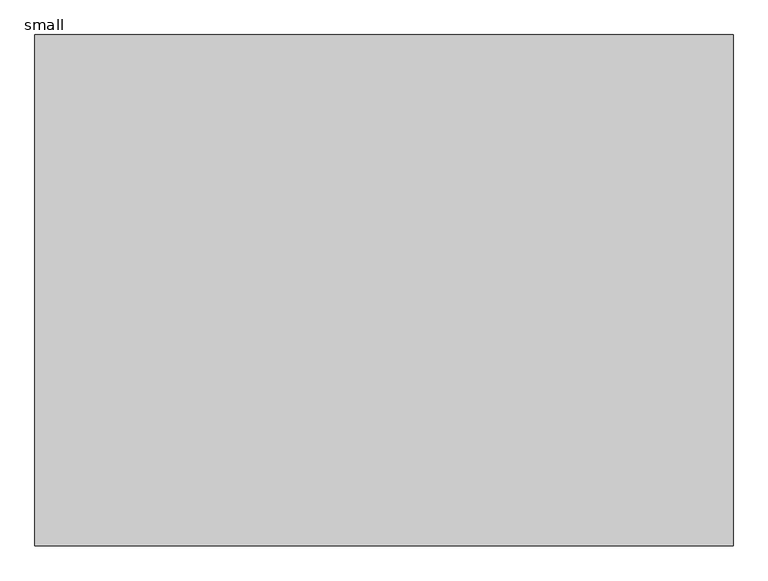
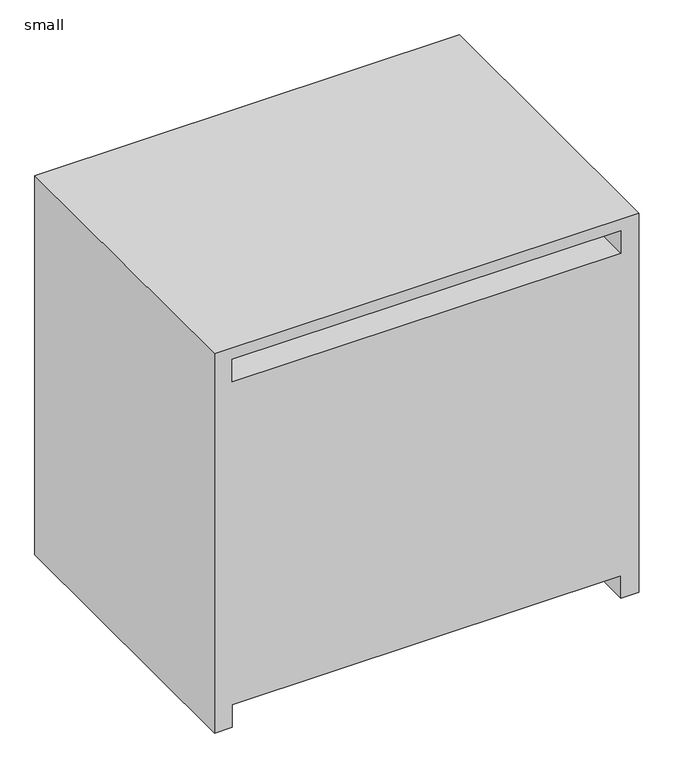
"""IFC4 building model written with IfcOpenShell, lengths in millimetres: proxy geometry, Transformer-Dry-Type-Siemens : small."""

import ifcopenshell
import ifcopenshell.guid

model = None  # the IFC model being written
_history = None  # IfcOwnerHistory: only IFC2X3 demands one
_inside = {}  # id of a spatial element -> (the spatial element, [elements in it])
_under = {}  # id of a project, library or spatial element -> (it, [spatial elements below it])
_declared = {}  # id of a project -> (the project, [libraries it declares])
_typed = {}  # id of a type object -> (the type object, [elements of that type])
_made_of = {}  # id of a material, layer set ... -> (it, [elements and type objects made of it])


def new_model(schema):
    """Start an empty IFC model of exactly this schema.

    Asked for "IFC4X3", IfcOpenShell would pick the latest addendum, in which some entities
    have other attributes; the version numbers below select the first issue.
    IFC2X3 requires an IfcOwnerHistory on every rooted entity: one is made here for all.
    """
    global model, _history
    if schema == "IFC4X3":
        model = ifcopenshell.file(schema_version=(4, 3, 0, 0))
    else:
        model = ifcopenshell.file(schema=schema)
    _inside.clear()
    _under.clear()
    _declared.clear()
    _typed.clear()
    _made_of.clear()
    _history = None
    if model.schema == "IFC2X3":
        org = make("IfcOrganization", Name="unknown")
        user = make(
            "IfcPersonAndOrganization",
            ThePerson=make("IfcPerson", FamilyName="unknown"),
            TheOrganization=org,
        )
        app = make(
            "IfcApplication",
            ApplicationDeveloper=org,
            Version="unknown",
            ApplicationFullName="unknown",
            ApplicationIdentifier="unknown",
        )
        _history = make(
            "IfcOwnerHistory",
            OwningUser=user,
            OwningApplication=app,
            ChangeAction="ADDED",
            CreationDate=0,
        )
    return model


def make(cls, **values):
    """One entity of the class cls with the attributes given. An attribute that is None is left unset."""
    return model.create_entity(
        cls, **{name: value for name, value in values.items() if value is not None}
    )


def rooted(cls, **values):
    """An entity with a GlobalId (a new one), such as an element, a storey or a relation."""
    return make(cls, GlobalId=ifcopenshell.guid.new(), OwnerHistory=_history, **values)


def si_unit(unit_type, name, prefix=None):
    """IfcSIUnit, for example si_unit("LENGTHUNIT", "METRE", prefix="MILLI")."""
    return make("IfcSIUnit", UnitType=unit_type, Prefix=prefix, Name=name)


def assignment(units):
    """IfcUnitAssignment: the units of a project."""
    return None if units is None else make("IfcUnitAssignment", Units=units)


def point(xyz):
    """IfcCartesianPoint."""
    return None if xyz is None else make("IfcCartesianPoint", Coordinates=xyz)


def direction(xyz):
    """IfcDirection."""
    return None if xyz is None else make("IfcDirection", DirectionRatios=xyz)


def frame(location, z_axis=None, x_axis=None):
    """IfcAxis2Placement3D, a coordinate frame: its origin and axes. An axis left out is left unset."""
    return make(
        "IfcAxis2Placement3D",
        Location=point(location),
        Axis=direction(z_axis),
        RefDirection=direction(x_axis),
    )


def origin():
    """The frame at (0, 0, 0) with its axes left unset."""
    return frame((0.0, 0.0, 0.0))


def place(relative_to, where):
    """IfcLocalPlacement: puts the frame where relative to a parent placement (None: the world)."""
    return make(
        "IfcLocalPlacement", PlacementRelTo=relative_to, RelativePlacement=where
    )


def context(
    kind, dimensions, precision=None, world=None, true_north=None, identifier=None
):
    """IfcGeometricRepresentationContext, for example the 3D "Model" context."""
    return make(
        "IfcGeometricRepresentationContext",
        ContextIdentifier=identifier,
        ContextType=kind,
        CoordinateSpaceDimension=dimensions,
        Precision=precision,
        WorldCoordinateSystem=world,
        TrueNorth=true_north,
    )


def project(units=None, contexts=None):
    """IfcProject with its units and contexts."""
    return rooted(
        "IfcProject",
        Name="project",
        RepresentationContexts=contexts,
        UnitsInContext=assignment(units),
    )


def spatial(cls, under=None, at=None, **own):
    """A site, building, storey or space (cls), placed at a placement, below another one or the project."""
    s = rooted(cls, ObjectPlacement=at, **own)
    if under is not None:
        _under.setdefault(under.id(), (under, []))[1].append(s)
    return s


def polyline(points):
    """IfcPolyline through the points."""
    return make("IfcPolyline", Points=[point(p) for p in points])


def outline(outer, holes=None, kind="AREA"):
    """IfcArbitraryClosedProfileDef: a profile drawn as a closed curve; with holes, ...WithVoids."""
    if holes is None:
        return make("IfcArbitraryClosedProfileDef", ProfileType=kind, OuterCurve=outer)
    return make(
        "IfcArbitraryProfileDefWithVoids",
        ProfileType=kind,
        OuterCurve=outer,
        InnerCurves=holes,
    )


def extrude(swept, where, along, depth):
    """IfcExtrudedAreaSolid: the profile swept, set in the frame where, extruded along a direction by depth."""
    return make(
        "IfcExtrudedAreaSolid",
        SweptArea=swept,
        Position=where,
        ExtrudedDirection=direction(along),
        Depth=depth,
    )


def shape(context_of_items, identifier, shape_type, items):
    """IfcShapeRepresentation: the items that make up one representation, for example the "Body"."""
    return make(
        "IfcShapeRepresentation",
        ContextOfItems=context_of_items,
        RepresentationIdentifier=identifier,
        RepresentationType=shape_type,
        Items=items,
    )


def source(mapping_origin, context_of_items, identifier, shape_type, items):
    """IfcRepresentationMap: a shape defined once, which mapped items show again and again."""
    return make(
        "IfcRepresentationMap",
        MappingOrigin=mapping_origin,
        MappedRepresentation=shape(context_of_items, identifier, shape_type, items),
    )


def transform(
    local_origin,
    x_axis=None,
    y_axis=None,
    z_axis=None,
    scale=None,
    scale2=None,
    scale3=None,
    uniform=True,
):
    """IfcCartesianTransformationOperator3D, or its non-uniform kind. x_axis, y_axis, z_axis: its Axis1, 2, 3."""
    if uniform:
        return make(
            "IfcCartesianTransformationOperator3D",
            Axis1=direction(x_axis),
            Axis2=direction(y_axis),
            LocalOrigin=point(local_origin),
            Scale=scale,
            Axis3=direction(z_axis),
        )
    return make(
        "IfcCartesianTransformationOperator3DnonUniform",
        Axis1=direction(x_axis),
        Axis2=direction(y_axis),
        LocalOrigin=point(local_origin),
        Scale=scale,
        Axis3=direction(z_axis),
        Scale2=scale2,
        Scale3=scale3,
    )


def mapped(mapping_source, mapping_target):
    """IfcMappedItem: shows the shape of a source again, moved by a transform."""
    return make(
        "IfcMappedItem", MappingSource=mapping_source, MappingTarget=mapping_target
    )


def made_of(thing, what):
    """Note that an element or type object is made of a material, layer set ...; save() writes the relation."""
    if what is not None:
        _made_of.setdefault(what.id(), (what, []))[1].append(thing)
    return thing


def element(
    cls,
    number,
    at=None,
    inside=None,
    cuts=None,
    type_object=None,
    material=None,
    context=None,
    identifier="Body",
    shape_type=None,
    held_by="IfcProductDefinitionShape",
    body=None,
    shapes=None,
    **own,
):
    """One element of the class cls, such as IfcWall. Its Tag is "e" and its number.

    at: its placement. inside: the storey or other place that contains it. cuts: it is an
    opening in that element (IfcRelVoidsElement). A single representation is given by context,
    identifier, shape_type and body (its items); several are given by shapes. held_by: the class
    of the entity that holds the representations. save() writes the other relations.
    """
    e = rooted(cls, Tag="e%d" % number, ObjectPlacement=at, **own)
    if body is not None:
        shapes = [shape(context, identifier, shape_type, body)]
    if shapes is not None:
        e.Representation = make(held_by, Representations=shapes)
    if inside is not None:
        _inside.setdefault(inside.id(), (inside, []))[1].append(e)
    if cuts is not None:
        rooted(
            "IfcRelVoidsElement", RelatingBuildingElement=cuts, RelatedOpeningElement=e
        )
    if type_object is not None:
        _typed.setdefault(type_object.id(), (type_object, []))[1].append(e)
    return made_of(e, material)


def aggregate(whole, parts):
    """IfcRelAggregates: a whole, such as a stair, and the parts it consists of."""
    return rooted("IfcRelAggregates", RelatingObject=whole, RelatedObjects=parts)


def save(model, path):
    """Write the relations noted so far, then the file.

    IfcRelAggregates (storeys below a building ...), IfcRelContainedInSpatialStructure (elements
    in a storey), IfcRelDefinesByType, IfcRelAssociatesMaterial and IfcRelDeclares: one each for
    every whole, place, type object, material and project.
    """
    for whole, parts in _under.values():
        aggregate(whole, parts)
    for where, things in _inside.values():
        rooted(
            "IfcRelContainedInSpatialStructure",
            RelatedElements=things,
            RelatingStructure=where,
        )
    for kind, things in _typed.values():
        rooted("IfcRelDefinesByType", RelatedObjects=things, RelatingType=kind)
    for what, things in _made_of.values():
        rooted("IfcRelAssociatesMaterial", RelatedObjects=things, RelatingMaterial=what)
    for by, libraries in _declared.values():
        rooted("IfcRelDeclares", RelatingContext=by, RelatedDefinitions=libraries)
    model.write(path)


def small_32f65543(model_context):
    return source(origin(), model_context, "Body", "SweptSolid", [
        extrude(outline(polyline([(1701.8, 901.7), (1701.8, -901.7), (0.0, -901.7), (0.0, -825.5), (101.6, -825.5), (101.6, 825.5), (0.0, 825.5), (0.0, 901.7), (1701.8, 901.7)]), holes=[polyline([(1651.0, 825.5), (1549.4, 825.5), (1549.4, -825.5), (1651.0, -825.5), (1651.0, 825.5)])]), frame((0.0, -660.4, 0.0), z_axis=(0.0, 1.0, 0.0), x_axis=(0.0, 0.0, 1.0)), (0.0, 0.0, 1.0), 1320.8),
    ])


if __name__ == "__main__":
    model = new_model("IFC4")
    model_context = context("Model", 3, world=origin())
    ifc_project = project(units=[si_unit("LENGTHUNIT", "METRE", prefix="MILLI")], contexts=[model_context])
    site = spatial("IfcSite", under=ifc_project)
    building = spatial("IfcBuilding", under=site)
    placement = place(None, origin())
    small_shape = small_32f65543(model_context)
    element("IfcBuildingElementProxy", 1, Name="Transformer-Dry-Type-Siemens : small", ObjectType="Transformer-Dry-Type-Siemens : small", at=placement, inside=building, context=model_context, shape_type="MappedRepresentation", body=[
        mapped(small_shape, transform((0.0, 0.0, 0.0), x_axis=(1.0, 0.0, 0.0), y_axis=(0.0, 1.0, 0.0), z_axis=(0.0, 0.0, 1.0))),
    ])
    save(model, "model.ifc")

# Revit data of these elements
# Type "Transformer-Dry-Type-Siemens : small"
#   Weight = "5500"
#   Wattage = "DO NOT USE"
#   Voltage = "DO NOT USE"
#   URL = "http://www.usa.siemens.com/ce"
#   Transformer Material = "Aluminum"
#   Product Page URL = "http://www.sea.siemens.com/us/Products/PowerDistribution/Product/Transformers/Pages/Transformers.aspx"
#   Product Documentation Link = "http://www.sea.siemens.com/us/internet-dms/Internet/ConsultingEngineersComm/General/Docs/drytrans.pdf"
#   Model = "3F3Y015K13TP1"
#   Manufacturer = "Siemens Industry"
#   KVA = "750"
#   K Factor = "13"
#   Description = "Transformer"
#   Deg Rise = "150"
#   Copyright © = "© Siemens Industry, Inc. 2011"
#   CTRL Connector Description = "Equipment Power"
#   BOM URL [instance default] = ""
#   Assembly Code = "D5090900"
#   clearance = 3' - 0"
#   Width = 5' - 11"
#   Primary Voltage = 480 V
#   Power Factor = 1
#   Height = 5' - 7"
#   Depth = 4' - 4"
#   Apparent Load [instance default] = 0 VA
#   Has Not Contacted Siemens For Configuration [instance default] = no
#   Contacted Siemens For Configuration [instance default] = yes
#   Text Material = Paint- Siemens - Dark
#   Frame Material = ELECTRICAL TRANSFORMERS
# Element 1 (IfcBuildingElementProxy, "Transformer-Dry-Type-Siemens : small")
#   Materials on its faces: "ELECTRICAL TRANSFORMERS"
# Materials
#   "Paint- Siemens - Dark": class "Metal", colour RGB 175 38 68, transparency 0
#   "ELECTRICAL TRANSFORMERS": class "Metal", colour RGB 63 114 97, transparency 0, Cost = 0
